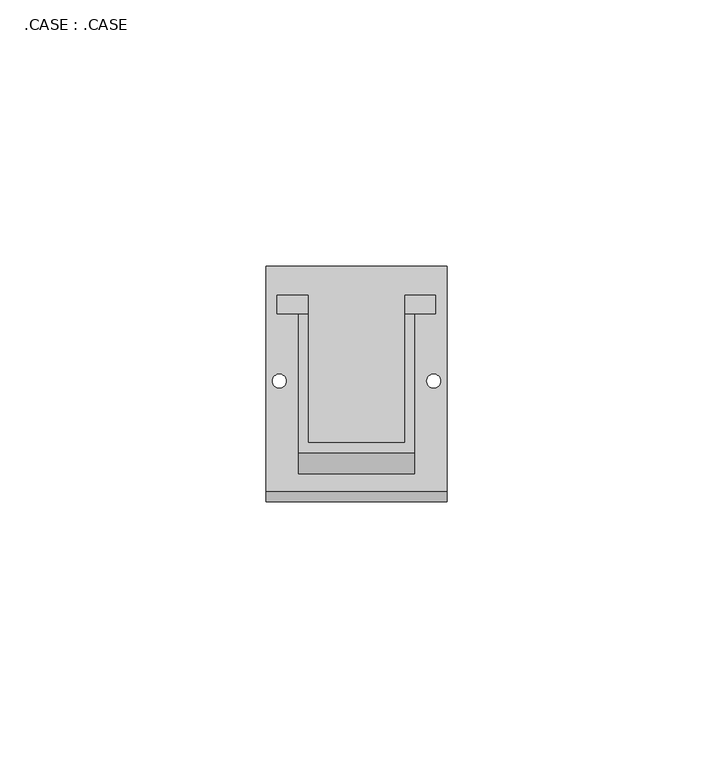
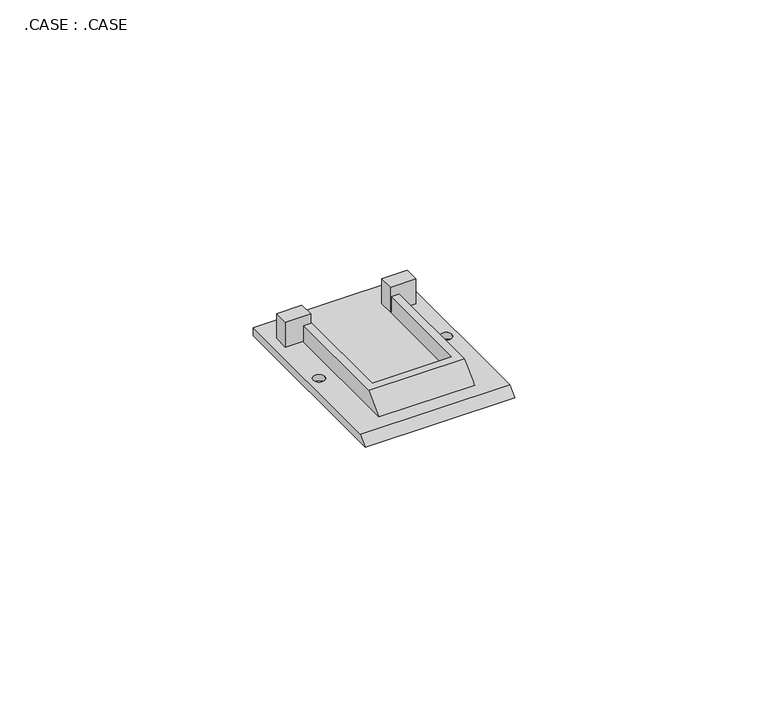
"""IFC4 building model written with IfcOpenShell, lengths in millimetres: proxy geometry, .CASE : .CASE."""

from ifc_helpers import new_model, si_unit, frame, origin, place, context, project, spatial, polyline, circle_curve, outline, extrude, source, transform, mapped, element, save
from ifc_brep_helpers import plane_surface, revolved_surface, advanced_brep


def case_case_ec59ddf9(model_context):
    return source(origin(), model_context, "Body", "SolidModel", [
        extrude(outline(polyline([(1461.1150176, 13229.1739696), (1466.9150176, 13229.1739696), (1466.9150176, 13225.7186096), (1461.1150176, 13225.7186096), (1461.1150176, 13229.1739696)])), frame((0.0, 0.0, 2.0), z_axis=(0.0, 0.0, 1.0), x_axis=(1.0, 0.0, 0.0)), (0.0, 0.0, 1.0), 6.0),
        extrude(outline(polyline([(1442.9350176, 13229.1739696), (1442.9350176, 13225.7186096), (1437.1350176, 13225.7186096), (1437.1350176, 13229.1739696), (1442.9350176, 13229.1739696)])), frame((0.0, 0.0, 2.0), z_axis=(0.0, 0.0, 1.0), x_axis=(1.0, 0.0, 0.0)), (0.0, 0.0, 1.0), 6.0),
        advanced_brep(
        [(1469.0250176, 13192.4212784, 2.0), (1469.0250176, 13234.6739696, 2.0), (1435.0250176, 13234.6739696, 2.0), (1435.0250176, 13192.4212784, 2.0), (1441.1350176, 13195.6739696, 2.0), (1441.1350176, 13225.7186096, 2.0), (1442.9350176, 13225.7186096, 2.0), (1442.9350176, 13201.4739696, 2.0), (1461.1150176, 13201.4739696, 2.0), (1461.1150176, 13225.7186096, 2.0), (1462.9150176, 13225.7186096, 2.0), (1462.9150176, 13195.6739696, 2.0), (1467.8250176, 13213.1041412, 2.0), (1465.2250176, 13213.1041412, 2.0), (1438.8250176, 13213.1041412, 2.0), (1436.2250176, 13213.1041412, 2.0), (1435.0250176, 13234.6739696, 0.0), (1469.0250176, 13234.6739696, 0.0), (1469.0250176, 13190.4212784, 0.0), (1435.0250176, 13190.4212784, 0.0), (1464.5250176, 13213.1041412, 0.0), (1468.5250176, 13213.1041412, 0.0), (1435.5250176, 13213.1041412, 0.0), (1439.5250176, 13213.1041412, 0.0), (1441.1350176, 13225.7186096, 6.0), (1441.1350176, 13199.6739696, 6.0), (1462.9150176, 13199.6739696, 6.0), (1462.9150176, 13225.7186096, 6.0), (1461.1150176, 13225.7186096, 6.0), (1461.1150176, 13201.4739696, 6.0), (1442.9350176, 13201.4739696, 6.0), (1442.9350176, 13225.7186096, 6.0)],
        [
            (0, 1),
            (1, 2),
            (2, 3),
            (3, 0),
            (4, 5),
            (5, 6),
            (6, 7),
            (7, 8),
            (8, 9),
            (9, 10),
            (10, 11),
            (11, 4),
            (12, 13, circle_curve(frame((1466.5250176, 13213.1041412, 2.0), z_axis=(0.0, 0.0, -1.0), x_axis=(-1.0, 0.0, 0.0)), 1.3)),
            (13, 12, circle_curve(frame((1466.5250176, 13213.1041412, 2.0), z_axis=(0.0, 0.0, -1.0), x_axis=(1.0, 0.0, 0.0)), 1.3)),
            (14, 15, circle_curve(frame((1437.5250176, 13213.1041412, 2.0), z_axis=(0.0, 0.0, -1.0), x_axis=(-1.0, 0.0, 0.0)), 1.3)),
            (15, 14, circle_curve(frame((1437.5250176, 13213.1041412, 2.0), z_axis=(0.0, 0.0, -1.0), x_axis=(1.0, 0.0, 0.0)), 1.3)),
            (16, 17),
            (17, 18),
            (18, 19),
            (19, 16),
            (20, 21, circle_curve(frame((1466.5250176, 13213.1041412, 0.0), z_axis=(0.0, 0.0, 1.0), x_axis=(-1.0, 0.0, 0.0)), 2.0)),
            (21, 20, circle_curve(frame((1466.5250176, 13213.1041412, 0.0), z_axis=(0.0, 0.0, 1.0), x_axis=(1.0, 0.0, 0.0)), 2.0)),
            (22, 23, circle_curve(frame((1437.5250176, 13213.1041412, 0.0), z_axis=(0.0, 0.0, 1.0), x_axis=(-1.0, 0.0, 0.0)), 2.0)),
            (23, 22, circle_curve(frame((1437.5250176, 13213.1041412, 0.0), z_axis=(0.0, 0.0, 1.0), x_axis=(1.0, 0.0, 0.0)), 2.0)),
            (0, 18),
            (17, 1),
            (16, 2),
            (19, 3),
            (24, 25),
            (25, 26),
            (26, 27),
            (27, 28),
            (28, 29),
            (29, 30),
            (30, 31),
            (31, 24),
            (24, 5),
            (4, 25),
            (26, 11),
            (10, 27),
            (9, 28),
            (8, 29),
            (7, 30),
            (6, 31),
            (20, 13),
            (12, 21),
            (22, 15),
            (14, 23),
        ],
        [
            plane_surface(frame((1467.7850176, 13192.4212784, 2.0), z_axis=(0.0, 0.0, 1.0), x_axis=(1.0, 0.0, 0.0))),
            plane_surface(frame((1467.7850176, 13192.4212784, 0.0), z_axis=(0.0, 0.0, -1.0), x_axis=(-1.0, 0.0, 0.0))),
            plane_surface(frame((1469.0250176, 13192.4212784, 2.0), z_axis=(1.0, 0.0, 0.0), x_axis=(0.0, 0.0, -1.0))),
            plane_surface(frame((1469.0250176, 13234.6739696, 2.0), z_axis=(0.0, 1.0, 0.0), x_axis=(0.0, 0.0, -1.0))),
            plane_surface(frame((1435.0250176, 13234.6739696, 2.0), z_axis=(-1.0, 0.0, 0.0), x_axis=(0.0, 0.0, -1.0))),
            plane_surface(frame((1441.1350176, 13234.6739696, 6.0), z_axis=(0.0, 0.0, 1.0), x_axis=(0.0, -1.0, 0.0))),
            plane_surface(frame((1441.1350176, 13225.7186096, 6.0), z_axis=(-1.0, 0.0, 0.0), x_axis=(0.0, 0.0, -1.0))),
            plane_surface(frame((1462.9150176, 13199.6739696, 6.0), z_axis=(1.0, 0.0, 0.0), x_axis=(0.0, 0.0, -1.0))),
            plane_surface(frame((1462.9150176, 13225.7186096, 6.0), z_axis=(0.0, 1.0, 0.0), x_axis=(0.0, 0.0, -1.0))),
            plane_surface(frame((1461.1150176, 13225.7186096, 6.0), z_axis=(-1.0, 0.0, 0.0), x_axis=(0.0, 0.0, -1.0))),
            plane_surface(frame((1461.1150176, 13201.4739696, 6.0), z_axis=(0.0, 1.0, 0.0), x_axis=(0.0, 0.0, -1.0))),
            plane_surface(frame((1442.9350176, 13201.4739696, 6.0), z_axis=(1.0, 0.0, 0.0), x_axis=(0.0, 0.0, -1.0))),
            plane_surface(frame((1442.9350176, 13225.7186096, 6.0), z_axis=(0.0, 1.0, 0.0), x_axis=(0.0, 0.0, -1.0))),
            plane_surface(frame((1441.1350176, 13195.6739696, 2.0), z_axis=(0.0, -0.7071067811865885, 0.7071067811865066), x_axis=(1.0, 0.0, 0.0))),
            plane_surface(frame((1435.0250176, 13190.4212784, 0.0), z_axis=(0.0, -0.707106781186628, 0.7071067811864672), x_axis=(1.0, 0.0, 0.0))),
            revolved_surface(polyline([(1464.5250176, 13213.1041412, 0.0), (1465.2250176017499, 13213.1041412, 2.0)]), (1466.5250176, 13213.1041412, 5.7142857), (0.0, 0.0, -1.0)),
            revolved_surface(polyline([(1435.5250176, 13213.1041412, 0.0), (1436.2250176017499, 13213.1041412, 2.0)]), (1437.5250176, 13213.1041412, 5.7142857), (0.0, 0.0, -1.0)),
        ],
        [
            (0, [[1, 2, 3, 4], [5, 6, 7, 8, 9, 10, 11, 12], [13, 14], [15, 16]]),
            (1, [[17, 18, 19, 20], [21, 22], [23, 24]]),
            (2, [[-1, 25, -18, 26]]),
            (3, [[-2, -26, -17, 27]]),
            (4, [[-3, -27, -20, 28]]),
            (5, [[29, 30, 31, 32, 33, 34, 35, 36]]),
            (6, [[-29, 37, -5, 38]]),
            (7, [[-31, 39, -11, 40]]),
            (8, [[-32, -40, -10, 41]]),
            (9, [[-33, -41, -9, 42]]),
            (10, [[-34, -42, -8, 43]]),
            (11, [[-35, -43, -7, 44]]),
            (12, [[-36, -44, -6, -37]]),
            (13, [[-38, -12, -39, -30]]),
            (14, [[-28, -19, -25, -4]]),
            (15, [[45, -13, 46, -21]]),
            (15, [[-45, -22, -46, -14]]),
            (16, [[47, -15, 48, -23]]),
            (16, [[-47, -24, -48, -16]]),
        ],
    ),
    ])


if __name__ == "__main__":
    model = new_model("IFC4")
    model_context = context("Model", 3, world=origin())
    ifc_project = project(units=[si_unit("LENGTHUNIT", "METRE", prefix="MILLI")], contexts=[model_context])
    site = spatial("IfcSite", under=ifc_project)
    building = spatial("IfcBuilding", under=site)
    placement = place(None, origin())
    case_case_shape = case_case_ec59ddf9(model_context)
    element("IfcBuildingElementProxy", 1, Name=".CASE : .CASE", ObjectType=".CASE : .CASE", at=placement, inside=building, context=model_context, shape_type="MappedRepresentation", body=[
        mapped(case_case_shape, transform((0.0, 0.0, 0.0), x_axis=(1.0, 0.0, 0.0), y_axis=(0.0, 1.0, 0.0), z_axis=(0.0, 0.0, 1.0))),
    ])
    save(model, "model.ifc")

# Revit data of these elements
# Project information
#   Data de emissão do projeto = "Data de emissão"
#   Status do projeto = "Status do projeto"
#   Nome do cliente = "Proprietário"
#   Endereço do projeto = "Insira aqui o endereço"
#   Nome do projeto = "Nome do projeto"
#   Número do projeto = "0001"
# Element 1 (IfcBuildingElementProxy, ".CASE : .CASE")
#   Materials on its faces: "Areia"
# Materials
#   "Areia": class "Genérico", colour RGB 191 183 178, transparency 0, Description = "Areia", Cost = 0
